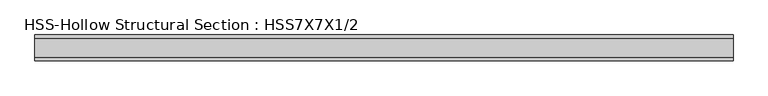
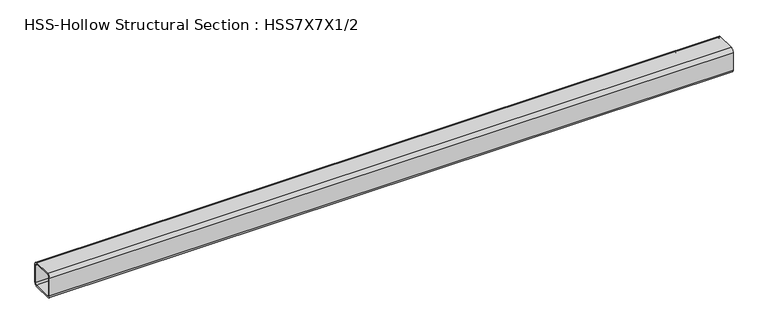
"""IFC4 building model written with IfcOpenShell, lengths in millimetres: member geometry, HSS-Hollow Structural Section : HSS7X7X1/2."""

from ifc_helpers import new_model, si_unit, point, frame, frame_2d, origin, place, context, project, spatial, polyline, circle_curve, trimmed, segment, composite_curve, outline, extrude, source, transform, mapped, element, save


def hss_hollow_structural_section_hss7x7x1_2_bde44d40(model_context):
    return source(origin(), model_context, "Body", "SweptSolid", [
        extrude(outline(composite_curve([segment(polyline([(88.9, 65.278), (88.9, -65.278)]), True, "CONTINUOUS"), segment(trimmed(circle_curve(frame_2d((65.278, -65.278)), 23.622), [point((88.9, -65.278))], [point((65.278, -88.9))], False, "CARTESIAN"), True, "CONTINUOUS"), segment(polyline([(65.278, -88.9), (-65.278, -88.9)]), True, "CONTINUOUS"), segment(trimmed(circle_curve(frame_2d((-65.278, -65.278)), 23.622), [point((-65.278, -88.9))], [point((-88.9, -65.278))], False, "CARTESIAN"), True, "CONTINUOUS"), segment(polyline([(-88.9, -65.278), (-88.9, 65.278)]), True, "CONTINUOUS"), segment(trimmed(circle_curve(frame_2d((-65.278, 65.278)), 23.622), [point((-88.9, 65.278))], [point((-65.278, 88.9))], False, "CARTESIAN"), True, "CONTINUOUS"), segment(polyline([(-65.278, 88.9), (65.278, 88.9)]), True, "CONTINUOUS"), segment(trimmed(circle_curve(frame_2d((65.278, 65.278)), 23.622), [point((65.278, 88.9))], [point((88.9, 65.278))], False, "CARTESIAN"), True, "CONTINUOUS")], self_intersect=False), holes=[composite_curve([segment(trimmed(circle_curve(frame_2d((-65.278, 65.278)), 11.811), [point((-65.278, 77.089))], [point((-77.089, 65.278))], True, "CARTESIAN"), True, "CONTINUOUS"), segment(polyline([(-77.089, 65.278), (-77.089, -65.278)]), True, "CONTINUOUS"), segment(trimmed(circle_curve(frame_2d((-65.278, -65.278)), 11.811), [point((-77.089, -65.278))], [point((-65.278, -77.089))], True, "CARTESIAN"), True, "CONTINUOUS"), segment(polyline([(-65.278, -77.089), (65.278, -77.089)]), True, "CONTINUOUS"), segment(trimmed(circle_curve(frame_2d((65.278, -65.278)), 11.811), [point((65.278, -77.089))], [point((77.089, -65.278))], True, "CARTESIAN"), True, "CONTINUOUS"), segment(polyline([(77.089, -65.278), (77.089, 65.278)]), True, "CONTINUOUS"), segment(trimmed(circle_curve(frame_2d((65.278, 65.278)), 11.811), [point((77.089, 65.278))], [point((65.278, 77.089))], True, "CARTESIAN"), True, "CONTINUOUS"), segment(polyline([(65.278, 77.089), (-65.278, 77.089)]), True, "CONTINUOUS")], self_intersect=False)]), frame((-2296.992995, 0.0, 0.0), z_axis=(1.0, 0.0, 0.0), x_axis=(0.0, 1.0, 0.0)), (0.0, 0.0, 1.0), 4825.1659156),
    ])


if __name__ == "__main__":
    model = new_model("IFC4")
    model_context = context("Model", 3, world=origin())
    ifc_project = project(units=[si_unit("LENGTHUNIT", "METRE", prefix="MILLI")], contexts=[model_context])
    site = spatial("IfcSite", under=ifc_project)
    building = spatial("IfcBuilding", under=site)
    placement = place(None, origin())
    hss_hollow_structural_section_hss7x7x1_2_shape = hss_hollow_structural_section_hss7x7x1_2_bde44d40(model_context)
    element("IfcMember", 1, ObjectType="HSS-Hollow Structural Section : HSS7X7X1/2", at=placement, inside=building, context=model_context, shape_type="MappedRepresentation", body=[
        mapped(hss_hollow_structural_section_hss7x7x1_2_shape, transform((0.0, 0.0, 0.0), x_axis=(1.0, 0.0, 0.0), y_axis=(0.0, 1.0, 0.0), z_axis=(0.0, 0.0, 1.0))),
    ])
    save(model, "model.ifc")

# Revit data of these elements
# Type "HSS-Hollow Structural Section : HSS7X7X1/2"
#   Assembly Code = "B10"
#   Shape = "Square"
#   W = 41.9
#   Ht = 0' - 7"
#   Length [instance default] = 5' - 0"
#   b = 0' - 7"
#   kr = 0' - 0.93"
#   t = 0' - 0.465"
#   A = 0.0805556 SF
#   Structural Material [instance default] = Steel ASTM A500, Grade B, Rectangular and Square
# Element 1 (IfcMember, "HSS-Hollow Structural Section : HSS7X7X1/2")
#   Materials on its faces: "Steel ASTM A500, Grade B, Rectangular and Square"
# Materials
#   "Steel ASTM A500, Grade B, Rectangular and Square": class "Metal", colour RGB 199 199 199, transparency 0, Description = "Carbon steel", Cost = 0
